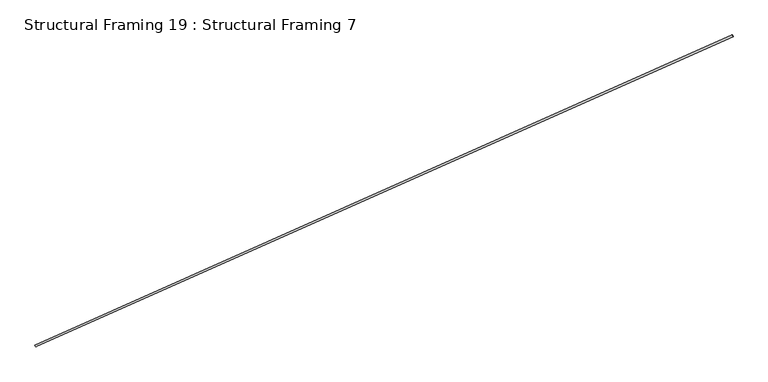
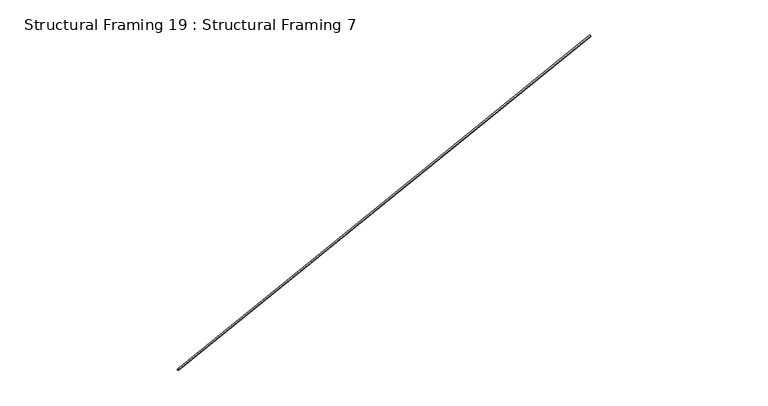
"""IFC4 building model written with IfcOpenShell, lengths in millimetres: beam geometry, Structural Framing 19 : Structural Framing 7."""

from ifc_helpers import new_model, si_unit, point, frame, origin, origin_2d, place, context, project, spatial, circle_curve, trimmed, segment, composite_curve, outline, extrude, source, transform, mapped, element, save


def structural_framing_19_structural_framing_7_32598720(model_context):
    return source(origin(), model_context, "Body", "SweptSolid", [
        extrude(outline(composite_curve([segment(trimmed(circle_curve(origin_2d(), 6.35), [point((-1e-07, -6.3500001))], [point((0.0, 6.35))], False, "CARTESIAN"), True, "CONTINUOUS"), segment(trimmed(circle_curve(origin_2d(), 6.35), [point((0.0, 6.35))], [point((-1e-07, -6.3500001))], False, "CARTESIAN"), True, "CONTINUOUS")], self_intersect=False)), frame((24994.3870052, 270.9973838, 2860.5759358), z_axis=(0.9135454576426018, 0.40642988240442374, 0.015793907347322014), x_axis=(0.0, 0.03883079534680305, -0.9992458002577418)), (0.0, 0.0, 1.0), 5505.1447719),
    ])


if __name__ == "__main__":
    model = new_model("IFC4")
    model_context = context("Model", 3, world=origin())
    ifc_project = project(units=[si_unit("LENGTHUNIT", "METRE", prefix="MILLI")], contexts=[model_context])
    site = spatial("IfcSite", under=ifc_project)
    building = spatial("IfcBuilding", under=site)
    placement = place(None, origin())
    structural_framing_19_structural_framing_7_shape = structural_framing_19_structural_framing_7_32598720(model_context)
    element("IfcBeam", 1, ObjectType="Structural Framing 19 : Structural Framing 7", at=placement, inside=building, context=model_context, shape_type="MappedRepresentation", body=[
        mapped(structural_framing_19_structural_framing_7_shape, transform((0.0, 0.0, 0.0), x_axis=(1.0, 0.0, 0.0), y_axis=(0.0, 1.0, 0.0), z_axis=(0.0, 0.0, 1.0))),
    ])
    save(model, "model.ifc")

# Revit data of these elements
# Type "Structural Framing 19 : Structural Framing 7"
#   Structural Material [instance default] = EXISTING LATERAL BRACING (1/4" CABLE)
# Element 1 (IfcBeam, "Structural Framing 19 : Structural Framing 7")
#   Materials on its faces: "EXISTING LATERAL BRACING (1/4\" CABLE)"
# Materials
#   "EXISTING LATERAL BRACING (1/4\" CABLE)": class "Generic", colour RGB 120 120 120, transparency 0, Cost = 0
